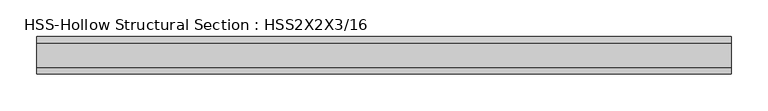
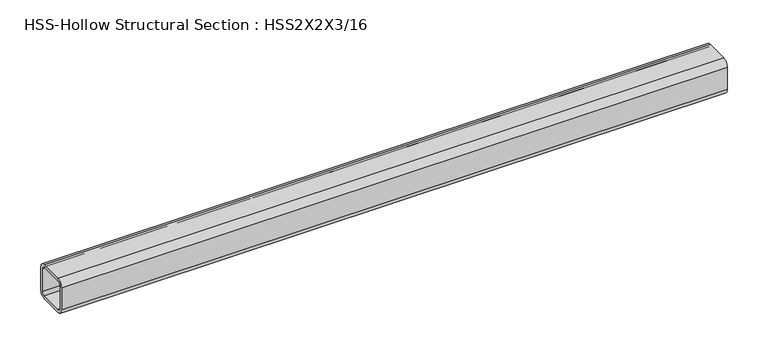
"""IFC4 building model written with IfcOpenShell, lengths in millimetres: beam geometry, HSS-Hollow Structural Section : HSS2X2X3/16."""

from ifc_helpers import new_model, si_unit, point, frame, frame_2d, origin, place, context, project, spatial, polyline, circle_curve, trimmed, segment, composite_curve, outline, extrude, source, transform, mapped, element, save


def hss_hollow_structural_section_hss2x2x3_16_095e06e8(model_context):
    return source(origin(), model_context, "Body", "SweptSolid", [
        extrude(outline(composite_curve([segment(polyline([(25.4, 16.5608), (25.4, -16.5608)]), True, "CONTINUOUS"), segment(trimmed(circle_curve(frame_2d((16.5608, -16.5608)), 8.8392), [point((25.4, -16.5608))], [point((16.5608, -25.4))], False, "CARTESIAN"), True, "CONTINUOUS"), segment(polyline([(16.5608, -25.4), (-16.5608, -25.4)]), True, "CONTINUOUS"), segment(trimmed(circle_curve(frame_2d((-16.5608, -16.5608)), 8.8392), [point((-16.5608, -25.4))], [point((-25.4, -16.5608))], False, "CARTESIAN"), True, "CONTINUOUS"), segment(polyline([(-25.4, -16.5608), (-25.4, 16.5608)]), True, "CONTINUOUS"), segment(trimmed(circle_curve(frame_2d((-16.5608, 16.5608)), 8.8392), [point((-25.4, 16.5608))], [point((-16.5608, 25.4))], False, "CARTESIAN"), True, "CONTINUOUS"), segment(polyline([(-16.5608, 25.4), (16.5608, 25.4)]), True, "CONTINUOUS"), segment(trimmed(circle_curve(frame_2d((16.5608, 16.5608)), 8.8392), [point((16.5608, 25.4))], [point((25.4, 16.5608))], False, "CARTESIAN"), True, "CONTINUOUS")], self_intersect=False), holes=[composite_curve([segment(trimmed(circle_curve(frame_2d((-16.5608, 16.5608)), 4.4196), [point((-16.5608, 20.9804))], [point((-20.9804, 16.5608))], True, "CARTESIAN"), True, "CONTINUOUS"), segment(polyline([(-20.9804, 16.5608), (-20.9804, -16.5608)]), True, "CONTINUOUS"), segment(trimmed(circle_curve(frame_2d((-16.5608, -16.5608)), 4.4196), [point((-20.9804, -16.5608))], [point((-16.5608, -20.9804))], True, "CARTESIAN"), True, "CONTINUOUS"), segment(polyline([(-16.5608, -20.9804), (16.5608, -20.9804)]), True, "CONTINUOUS"), segment(trimmed(circle_curve(frame_2d((16.5608, -16.5608)), 4.4196), [point((16.5608, -20.9804))], [point((20.9804, -16.5608))], True, "CARTESIAN"), True, "CONTINUOUS"), segment(polyline([(20.9804, -16.5608), (20.9804, 16.5608)]), True, "CONTINUOUS"), segment(trimmed(circle_curve(frame_2d((16.5608, 16.5608)), 4.4196), [point((20.9804, 16.5608))], [point((16.5608, 20.9804))], True, "CARTESIAN"), True, "CONTINUOUS"), segment(polyline([(16.5608, 20.9804), (-16.5608, 20.9804)]), True, "CONTINUOUS")], self_intersect=False)]), frame((8547.89375, 0.0, 0.0), z_axis=(1.0, 0.0, 0.0), x_axis=(0.0, 1.0, 0.0)), (0.0, 0.0, 1.0), 941.3875),
    ])


if __name__ == "__main__":
    model = new_model("IFC4")
    model_context = context("Model", 3, world=origin())
    ifc_project = project(units=[si_unit("LENGTHUNIT", "METRE", prefix="MILLI")], contexts=[model_context])
    site = spatial("IfcSite", under=ifc_project)
    building = spatial("IfcBuilding", under=site)
    placement = place(None, origin())
    hss_hollow_structural_section_hss2x2x3_16_shape = hss_hollow_structural_section_hss2x2x3_16_095e06e8(model_context)
    element("IfcBeam", 1, ObjectType="HSS-Hollow Structural Section : HSS2X2X3/16", at=placement, inside=building, context=model_context, shape_type="MappedRepresentation", body=[
        mapped(hss_hollow_structural_section_hss2x2x3_16_shape, transform((0.0, 0.0, 0.0), x_axis=(1.0, 0.0, 0.0), y_axis=(0.0, 1.0, 0.0), z_axis=(0.0, 0.0, 1.0))),
    ])
    save(model, "model.ifc")

# Revit data of these elements
# Type "HSS-Hollow Structural Section : HSS2X2X3/16"
#   Keynote = "M05121300.04"
#   Assembly Code = "B10"
#   Shape = "Square"
#   W = 4.3
#   Ht = 0' - 2"
#   Length [instance default] = 5' - 0"
#   b = 0' - 2"
#   kr = 0' - 0.348"
#   t = 0' - 0.174"
#   A = 0.00826389 SF
#   Structural Material [instance default] = Steel ASTM A500, Grade B, Rectangular and Square
# Element 1 (IfcBeam, "HSS-Hollow Structural Section : HSS2X2X3/16")
#   Materials on its faces: "Steel ASTM A500, Grade B, Rectangular and Square"
# Materials
#   "Steel ASTM A500, Grade B, Rectangular and Square": class "Metal", colour RGB 199 199 199, transparency 0, Description = "Carbon steel", Cost = 0
